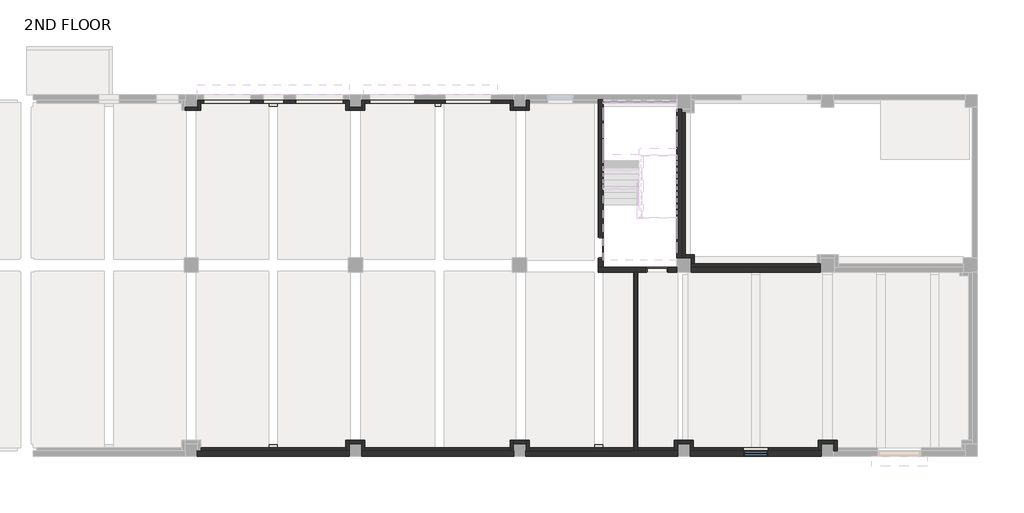
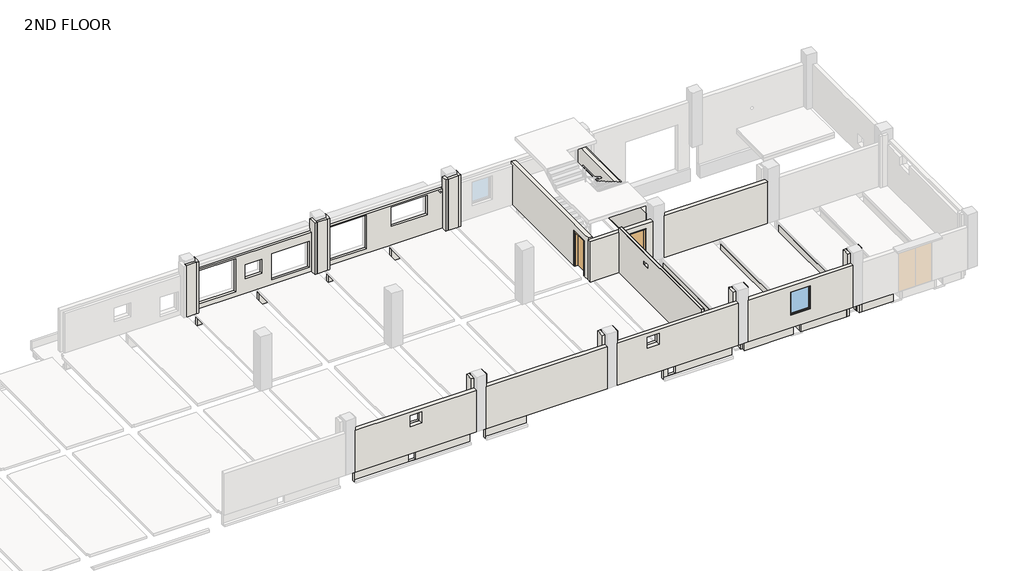
# One storey, part 2 of 7: 60 walls, 2 doors, 1 window.
# Revit data of these elements (continued)
# Type "Single Door_Steel : H_DR_AR B12_Door_Single_W1100xH2280_FR 1.0H_FSD-1" (continued)
#   Define Thermal Properties by = 1
#   문 패널 = none
#   문 프레임 = none
#   Function = (empty or 0)
#   Wall Closure = (empty or 0)
# Type "H_WA_AR B02_Ext Wall RC-AG_T250_W1"
#   Type Comments = "CV-AG"
#   H_Rebar Ratio = 0.12
#   Layers, outside or top first: 250 mm "Concrete_f'c=28MPa(Cylender)" (function 1)
# Type "H_WA_AR B02_Int Wall RC-AG_T250_W2"
#   Type Comments = "CV-AG"
#   H_Rebar Ratio = 0.12
#   Layers, outside or top first: 250 mm "Concrete_f'c=28MPa(Cylender)" (function 1)
# Type "H_WA_AR B02_Ext Wall DY-IN_T154"
#   Type Comments = ""
#   Layers, outside or top first: 0 mm "00_Finish_Paint_Vinyl Paint" (function 100); 9.5 mm "00_Finish_Gypsum Board" (function 4); 9.5 mm "00_Finish_Gypsum Board" (function 4); 135 mm "00_Insulation_Glass Wool" (function 3); 0 mm no material (function 100)
# Type "H_WA_AR B02_Int Wall MA_T150"
#   Type Comments = ""
#   Layers, outside or top first: 0 mm no material (function 100); 150 mm "00_Masonry_Conc. Block" (function 1); 0 mm no material (function 100)
# Type "H_WA_AR_B07_Int Wall_Plaster_T18"
#   Type Comments = ""
#   Layers, outside or top first: 18 mm "00_Finish_Plaster" (function 4)
# Type "H_CE_AR_B09_Souns Absorbing_100T_C7"
#   Type Comments = "finish"
#   Layers, outside or top first: 100 mm "00.Ceiling_Sound Absorbing" (function 4)
# Type "H_CE_AR_B09_Souns Absorbing_100T_C7 2"
#   Type Comments = "finish"
#   Layers, outside or top first: 164 mm "00.Ceiling_Sound Absorbing" (function 4)
# Type "Fixed Window : H_WD_AR_B11_Fix_Steel Window_SG_W1200xH1500_AW-2"
#   Type Mark = "269"
#   Analytic Construction = "<None>"
#   창 두께 = 150 mm
#   Height = 1500 mm
#   절반 창 두께 = 75 mm
#   기본 씰 높이 = 800 mm
#   Width = 1200 mm
#   ▽ = yes
#   Define Thermal Properties by = 1
#   창 패널 = none
#   창 프레임 = none
#   Wall Closure = (empty or 0)
#   Description = (empty or 0)
# Elements 1, 2 (IfcDoor, "Single Door_Steel : H_DR_AR B12_Door_Single_W1100xH2280_FR 1.0H_FSD-1")
#   Phase Created = New Construction
# Elements 3, 4, 5, 6 (IfcWall, "H_WA_AR B02_Ext Wall RC-AG_T250_W1")
#   Comments = ""
#   Top Offset = -800 mm
#   Base Offset = 0 mm
#   wall height = 2700 mm
#   Phase Created = New Construction
#   Base Constraint = 2ND FLOOR
#   Top Constraint = 3RD FLOOR
#   Materials on its faces: "Concrete_f'c=28MPa(Cylender)"
# Element 7 (IfcWall, "H_WA_AR B02_Int Wall RC-AG_T250_W2")
#   Comments = ""
#   Top Offset = -900 mm
#   Base Offset = 0 mm
#   wall height = 2600 mm
#   Phase Created = New Construction
#   Base Constraint = 2ND FLOOR
#   Top Constraint = 3RD FLOOR
#   Materials on its faces: "Concrete_f'c=28MPa(Cylender)"
# Elements 8, 9, 10 (IfcWall, "H_WA_AR B02_Int Wall RC-AG_T250_W2")
#   Comments = ""
#   Top Offset = -800 mm
#   Base Offset = 0 mm
#   wall height = 2700 mm
#   Phase Created = New Construction
#   Base Constraint = 2ND FLOOR
#   Top Constraint = 3RD FLOOR
#   Materials on its faces: "Concrete_f'c=28MPa(Cylender)"
# Elements 11, 15, 19, 23, 25 (IfcWall, "H_WA_AR B02_Ext Wall DY-IN_T154")
#   Top Offset = -945 mm
#   Base Offset = 0 mm
#   wall height = 2555 mm
#   Phase Created = New Construction
#   Base Constraint = 2ND FLOOR
#   Top Constraint = 3RD FLOOR
#   Materials on its faces: "Default Wall", "00_Insulation_Glass Wool", "00_Finish_Gypsum Board"
# Elements 12, 14, 16, 18, 20, 22, 26 (IfcWall, "H_WA_AR B02_Ext Wall DY-IN_T154")
#   Top Offset = -180 mm
#   Base Offset = 0 mm
#   wall height = 3320 mm
#   Phase Created = New Construction
#   Base Constraint = 2ND FLOOR
#   Top Constraint = 3RD FLOOR
#   Materials on its faces: "00_Insulation_Glass Wool", "00_Finish_Gypsum Board", "Default Wall"
# Elements 13, 17, 21, 27 (IfcWall, "H_WA_AR B02_Ext Wall DY-IN_T154")
#   Top Offset = -180 mm
#   Base Offset = 0 mm
#   wall height = 3320 mm
#   Phase Created = New Construction
#   Base Constraint = 2ND FLOOR
#   Top Constraint = 3RD FLOOR
#   Materials on its faces: "Default Wall", "00_Insulation_Glass Wool", "00_Finish_Gypsum Board"
# Element 24 (IfcWall, "H_WA_AR B02_Int Wall MA_T150")
#   Top Offset = -600 mm
#   Base Offset = 0 mm
#   wall height = 2900 mm
#   Phase Created = New Construction
#   Base Constraint = 2ND FLOOR
#   Top Constraint = 3RD FLOOR
#   Materials on its faces: "Default Wall", "00_Masonry_Conc. Block"
# Elements 28, 36 (IfcWall, "H_WA_AR B02_Ext Wall DY-IN_T154")
#   Top Offset = -180 mm
#   Base Offset = 0 mm
#   wall height = 3320 mm
#   Phase Created = New Construction
#   Base Constraint = 2ND FLOOR
#   Top Constraint = 3RD FLOOR
#   Materials on its faces: "00_Insulation_Glass Wool", "Default Wall", "00_Finish_Gypsum Board"
# Elements 29, 33, 37 (IfcWall, "H_WA_AR B02_Ext Wall DY-IN_T154")
#   Top Offset = -180 mm
#   Base Offset = 0 mm
#   wall height = 3320 mm
#   Phase Created = New Construction
#   Base Constraint = 2ND FLOOR
#   Top Constraint = 3RD FLOOR
#   Materials on its faces: "Default Wall", "00_Finish_Gypsum Board", "00_Insulation_Glass Wool"
# Elements 30, 32, 34, 38 (IfcWall, "H_WA_AR B02_Ext Wall DY-IN_T154")
#   Top Offset = -180 mm
#   Base Offset = 0 mm
#   wall height = 3320 mm
#   Phase Created = New Construction
#   Base Constraint = 2ND FLOOR
#   Top Constraint = 3RD FLOOR
#   Materials on its faces: "00_Finish_Gypsum Board", "00_Insulation_Glass Wool", "Default Wall"
# Elements 31, 35 (IfcWall, "H_WA_AR B02_Ext Wall DY-IN_T154")
#   Top Offset = -945 mm
#   Base Offset = 0 mm
#   wall height = 2555 mm
#   Phase Created = New Construction
#   Base Constraint = 2ND FLOOR
#   Top Constraint = 3RD FLOOR
#   Materials on its faces: "Default Wall", "00_Finish_Gypsum Board", "00_Insulation_Glass Wool"
# Elements 39, 42 (IfcWall, "H_WA_AR B02_Ext Wall DY-IN_T154")
#   built-in parameter 1001111 = 135 mm
#   Top Offset = -945 mm
#   Base Offset = 135 mm
#   wall height = 2420 mm
#   Phase Created = New Construction
#   Base Constraint = 2ND FLOOR
#   Top Constraint = 3RD FLOOR
#   Materials on its faces: "Default Wall", "00_Insulation_Glass Wool", "00_Finish_Gypsum Board"
# Element 40 (IfcWall, "H_WA_AR B02_Ext Wall DY-IN_T154")
#   Top Offset = -334 mm
#   Base Offset = 0 mm
#   wall height = 3166 mm
#   Phase Created = New Construction
#   Base Constraint = 2ND FLOOR
#   Top Constraint = 3RD FLOOR
#   Materials on its faces: "Default Wall", "00_Finish_Gypsum Board", "00_Insulation_Glass Wool"
# Element 41 (IfcWall, "H_WA_AR B02_Ext Wall DY-IN_T154")
#   Top Offset = -334 mm
#   Base Offset = 0 mm
#   wall height = 3166 mm
#   Phase Created = New Construction
#   Base Constraint = 2ND FLOOR
#   Top Constraint = 3RD FLOOR
#   Materials on its faces: "Default Wall", "00_Insulation_Glass Wool", "00_Finish_Gypsum Board"
# Element 43 (IfcWall, "H_WA_AR B02_Ext Wall DY-IN_T154")
#   built-in parameter 1001111 = -935 mm
#   Top Offset = 135 mm
#   Base Offset = -935 mm
#   wall height = 1070 mm
#   Phase Created = New Construction
#   Base Constraint = 2ND FLOOR
#   Top Constraint = 2ND FLOOR
#   Materials on its faces: "Default Wall", "00_Insulation_Glass Wool", "00_Finish_Gypsum Board"
# Elements 44, 45 (IfcWall, "H_WA_AR_B07_Int Wall_Plaster_T18")
#   Top Offset = -600 mm
#   Base Offset = 0 mm
#   wall height = 2900 mm
#   Phase Created = New Construction
#   Base Constraint = 2ND FLOOR
#   Top Constraint = 3RD FLOOR
#   Materials on its faces: "00_Finish_Plaster"
# Elements 46, 47, 49, 50, 51, 54, 55, 56 (IfcWall, "H_CE_AR_B09_Souns Absorbing_100T_C7")
#   built-in parameter 1001111 = -800 mm
#   Top Offset = -250 mm
#   Base Offset = -800 mm
#   wall height = 550 mm
#   Phase Created = New Construction
#   Base Constraint = 2ND FLOOR
#   Top Constraint = 2ND FLOOR
#   Materials on its faces: "00.Ceiling_Sound Absorbing"
# Elements 48, 52, 53 (IfcWall, "H_CE_AR_B09_Souns Absorbing_100T_C7 2")
#   built-in parameter 1001111 = -800 mm
#   Top Offset = -250 mm
#   Base Offset = -800 mm
#   wall height = 550 mm
#   Phase Created = New Construction
#   Base Constraint = 2ND FLOOR
#   Top Constraint = 2ND FLOOR
#   Materials on its faces: "00.Ceiling_Sound Absorbing"
# Elements 57, 58, 59 (IfcWall, "H_WA_AR B02_Ext Wall DY-IN_T154")
#   built-in parameter 1001111 = -945 mm
#   Top Offset = -150 mm
#   Base Offset = -945 mm
#   wall height = 795 mm
#   Phase Created = New Construction
#   Base Constraint = 2ND FLOOR
#   Top Constraint = 2ND FLOOR
#   Materials on its faces: "Default Wall", "00_Insulation_Glass Wool", "00_Finish_Gypsum Board"
# Elements 60, 61, 62 (IfcWall, "H_WA_AR B02_Ext Wall DY-IN_T154")
#   built-in parameter 1001111 = -945 mm
#   Top Offset = -150 mm
#   Base Offset = -945 mm
#   wall height = 795 mm
#   Phase Created = New Construction
#   Base Constraint = 2ND FLOOR
#   Top Constraint = 2ND FLOOR
#   Materials on its faces: "Default Wall", "00_Finish_Gypsum Board", "00_Insulation_Glass Wool"
# Element 63 (IfcWindow, "Fixed Window : H_WD_AR_B11_Fix_Steel Window_SG_W1200xH1500_AW-2")
#   Mark = "FRW-15"
#   Phase Created = New Construction
#   Materials on its faces: "00_Metal_Aluminum", "Glass"
# Materials
#   "Concrete_f'c=28MPa(Cylender)": class "Concrete", colour RGB 176 176 176, transparency 0, Description = "Reinf. Conc.", Cost = 0, Image = Concrete.Cast-In-Place.Flat.Polished.Grey.jpg
#   "00_Finish_Paint_Vinyl Paint": class "Finish", colour RGB 128 128 64, transparency 0, Description = "Plastic", Cost = 0
#   "00_Finish_Gypsum Board": class "Finish", colour RGB 171 170 168, transparency 0, Description = "Gypsum Board", Cost = 0, Image = Finishes.Gypsum Board.Painted.White.jpg
#   "00_Insulation_Glass Wool": class "Insulation", colour RGB 200 200 140, transparency 0, Description = "Insulation(Loose)", Cost = 0
#   "00_Masonry_Conc. Block": class "Concrete", colour RGB 180 180 180, transparency 0, Description = "Conc. Block", Cost = 0, Image = Brick_Uniform_12inch_Running_Gray.png
#   "00_Finish_Plaster": class "Finish", colour RGB 228 228 228, transparency 0, Description = "Gypsum Board", Cost = 0
#   "00.Ceiling_Sound Absorbing": class "Generic", colour RGB 100 102 90, transparency 0, Description = "Acoustic ceiling tile", Cost = 0
#   "Default Wall": class "Miscellaneous", colour RGB 80 80 80, transparency 0
#   "00_Metal_Aluminum": class "Metal", colour RGB 244 244 244, transparency 0, Description = "Aluminum", Cost = 0, Image = none
#   "Glass": class "Glass", colour RGB 218 227 224, transparency 0.85, Description = "Soda Lime Glass", Cost = 0
